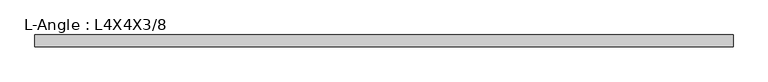
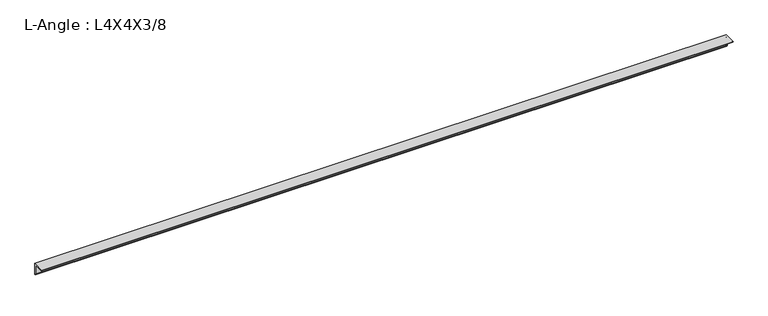
"""IFC4 building model written with IfcOpenShell, lengths in millimetres: beam geometry, L-Angle : L4X4X3/8."""

from ifc_helpers import new_model, si_unit, point, frame, frame_2d, origin, place, context, project, spatial, polyline, circle_curve, trimmed, segment, composite_curve, outline, extrude, source, transform, mapped, element, save


def l_angle_l4x4x3_8_c668a122(model_context):
    return source(origin(), model_context, "Body", "SweptSolid", [
        extrude(outline(composite_curve([segment(polyline([(28.702, 28.702), (28.702, -72.898)]), True, "CONTINUOUS"), segment(trimmed(circle_curve(frame_2d((28.702, -63.373)), 9.525), [point((28.702, -72.898))], [point((19.177, -63.373))], False, "CARTESIAN"), True, "CONTINUOUS"), segment(polyline([(19.177, -63.373), (19.177, 9.652)]), True, "CONTINUOUS"), segment(trimmed(circle_curve(frame_2d((9.652, 9.652)), 9.525), [point((19.177, 9.652))], [point((9.652, 19.177))], True, "CARTESIAN"), True, "CONTINUOUS"), segment(polyline([(9.652, 19.177), (-63.373, 19.177)]), True, "CONTINUOUS"), segment(trimmed(circle_curve(frame_2d((-63.373, 28.702)), 9.525), [point((-63.373, 19.177))], [point((-72.898, 28.702))], False, "CARTESIAN"), True, "CONTINUOUS"), segment(polyline([(-72.898, 28.702), (28.702, 28.702)]), True, "CONTINUOUS")], self_intersect=False)), frame((-2997.2, 0.0, 0.0), z_axis=(1.0, 0.0, 0.0), x_axis=(0.0, 1.0, 0.0)), (0.0, 0.0, 1.0), 6070.5999994),
    ])


if __name__ == "__main__":
    model = new_model("IFC4")
    model_context = context("Model", 3, world=origin())
    ifc_project = project(units=[si_unit("LENGTHUNIT", "METRE", prefix="MILLI")], contexts=[model_context])
    site = spatial("IfcSite", under=ifc_project)
    building = spatial("IfcBuilding", under=site)
    placement = place(None, origin())
    l_angle_l4x4x3_8_shape = l_angle_l4x4x3_8_c668a122(model_context)
    element("IfcBeam", 1, ObjectType="L-Angle : L4X4X3/8", at=placement, inside=building, context=model_context, shape_type="MappedRepresentation", body=[
        mapped(l_angle_l4x4x3_8_shape, transform((0.0, 0.0, 0.0), x_axis=(1.0, 0.0, 0.0), y_axis=(0.0, 1.0, 0.0), z_axis=(0.0, 0.0, 1.0))),
    ])
    save(model, "model.ifc")

# Revit data of these elements
# Type "L-Angle : L4X4X3/8"
#   Assembly Code = "B10"
#   k = 0' - 0 3/4"
#   W = 9.8
#   Length [instance default] = 5' - 0"
#   b = 0' - 4"
#   d = 0' - 4"
#   t = 0' - 0 3/8"
#   x = 0' - 1.13"
#   y = 0' - 1.13"
#   A = 0.0198611 SF
#   Structural Material [instance default] = Steel ASTM A36
# Element 1 (IfcBeam, "L-Angle : L4X4X3/8")
#   Materials on its faces: "Steel ASTM A36"
# Materials
#   "Steel ASTM A36": class "Metal", colour RGB 199 199 199, transparency 0, Description = "Structural steel, ASTM A36 Grade B, mill finish", Cost = 0
